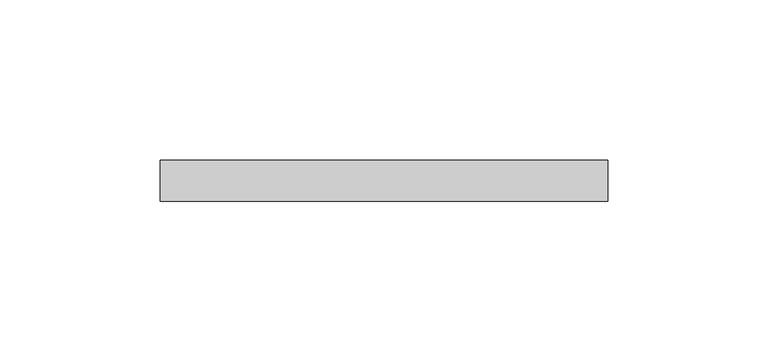
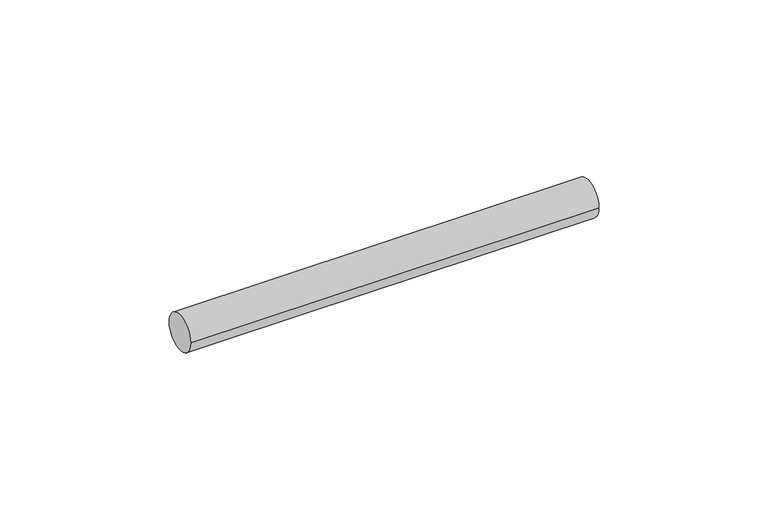
"""IFC4 building model written with IfcOpenShell, lengths in millimetres: proxy geometry, Generic Models 7:Generic Models 1:8:Generic Models 1:8 : Generic Models 7:Generic Models 1:337419:2 : Generic Models 7:Generic Models 1:8:Generic Models 1:8 : Generic Models 7:Generic Models 1:337419:315935."""

from ifc_helpers import new_model, si_unit, point, frame, frame_2d, origin, place, context, project, spatial, circle_curve, trimmed, segment, composite_curve, outline, extrude, source, transform, mapped, element, save


def generic_models_c66911f5(model_context):
    return source(origin(), model_context, "Body", "SweptSolid", [
        extrude(outline(composite_curve([segment(trimmed(circle_curve(frame_2d((-564919.104849, 8844.5106637)), 6.35), [point((-564912.754849, 8844.5106637))], [point((-564925.454849, 8844.5106637))], False, "CARTESIAN"), True, "CONTINUOUS"), segment(trimmed(circle_curve(frame_2d((-564919.104849, 8844.5106637)), 6.35), [point((-564925.454849, 8844.5106637))], [point((-564912.754849, 8844.5106637))], False, "CARTESIAN"), True, "CONTINUOUS")], self_intersect=False)), frame((593665.2601618, 0.0, 0.0), z_axis=(1.0, 0.0, 0.0), x_axis=(0.0, 1.0, 0.0)), (0.0, 0.0, 1.0), 139.3031242),
    ])


if __name__ == "__main__":
    model = new_model("IFC4")
    model_context = context("Model", 3, world=origin())
    ifc_project = project(units=[si_unit("LENGTHUNIT", "METRE", prefix="MILLI")], contexts=[model_context])
    site = spatial("IfcSite", under=ifc_project)
    building = spatial("IfcBuilding", under=site)
    placement = place(None, origin())
    generic_models_shape = generic_models_c66911f5(model_context)
    element("IfcBuildingElementProxy", 1, Name="Generic Models 7:Generic Models 1:8:Generic Models 1:8 : Generic Models 7:Generic Models 1:337419:2 : Generic Models 7:Generic Models 1:8:Generic Models 1:8 : Generic Models 7:Generic Models 1:337419:315935", ObjectType="Generic Models 7:Generic Models 1:8:Generic Models 1:8 : Generic Models 7:Generic Models 1:337419:2 : Generic Models 7:Generic Models 1:8:Generic Models 1:8 : Generic Models 7:Generic Models 1:337419:315935", at=placement, inside=building, context=model_context, shape_type="MappedRepresentation", body=[
        mapped(generic_models_shape, transform((0.0, 0.0, 0.0), x_axis=(1.0, 0.0, 0.0), y_axis=(0.0, 1.0, 0.0), z_axis=(0.0, 0.0, 1.0))),
    ])
    save(model, "model.ifc")

# Revit data of these elements
# Type "Generic Models 7:Generic Models 1:8:Generic Models 1:8 : Generic Models 7:Generic Models 1:337419:2 : Generic Models 7:Generic Models 1:8:Generic Models 1:8 : Generic Models 7:Generic Models 1:337419:315935"
#   NameOverride = "Generic Models 7:Generic Models 1:8:Generic Models 1:8 : Generic Models 7:Generic Models 1:337419:315935"
#   ObjectTypeOverride = "Generic Models 1:8 : Generic Models 7:Generic Models 1:337419"
#   Reference = "Generic Models 1"
#   Tag = "315935"
# Element 1 (IfcBuildingElementProxy, "Generic Models 7:Generic Models 1:8:Generic Models 1:8 : Generic Models 7:Generic Models 1:337419:2 : Generic Models 7:Generic Models 1:8:Generic Models 1:8 : Generic Models 7:Generic Models 1:337419:315935")
#   Materials on its faces: "0.179\" THICK BENT STEEL CLIPS"
# Materials
#   "0.179\" THICK BENT STEEL CLIPS": class "Metal", colour RGB 189 187 185, transparency 0, Description = "Structural steel 50ksi", Cost = 0
